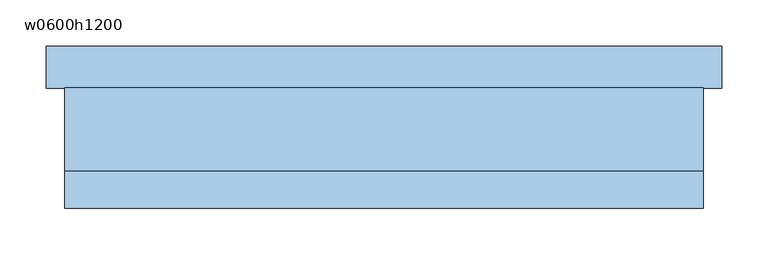
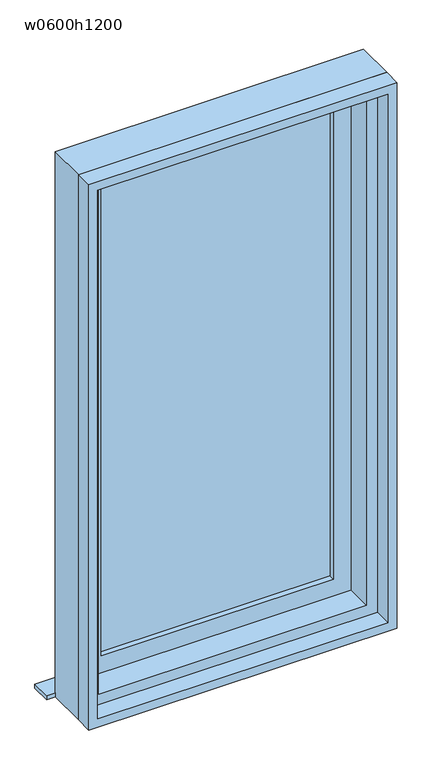
"""IFC4 building model written with IfcOpenShell, lengths in millimetres: window geometry, 縦すべり窓 : w0600h1200."""

from ifc_helpers import new_model, si_unit, frame, origin, place, context, project, spatial, polyline, outline, extrude, source, transform, mapped, element, save


def w0600h1200_ca4a6b53(model_context):
    return source(origin(), model_context, "Body", "SweptSolid", [
        extrude(outline(polyline([(260.0, 27.5), (-260.0, 27.5), (-260.0, 32.5), (260.0, 32.5), (260.0, 27.5)])), frame((0.0, 0.0, 840.0), z_axis=(0.0, 0.0, 1.0), x_axis=(1.0, 0.0, 0.0)), (0.0, 0.0, 1.0), 1120.0),
        extrude(outline(polyline([(2000.0, 300.0), (2000.0, -300.0), (800.0, -300.0), (800.0, 300.0), (2000.0, 300.0)]), holes=[polyline([(1960.0, -260.0), (1960.0, 260.0), (840.0, 260.0), (840.0, -260.0), (1960.0, -260.0)])]), frame((0.0, 15.0, 0.0), z_axis=(0.0, 1.0, 0.0), x_axis=(0.0, 0.0, 1.0)), (0.0, 0.0, 1.0), 30.0),
        extrude(outline(polyline([(365.0, 90.0), (365.0, 45.0), (-365.0, 45.0), (-365.0, 90.0), (365.0, 90.0)])), frame((0.0, 0.0, 755.0), z_axis=(0.0, 0.0, 1.0), x_axis=(1.0, 0.0, 0.0)), (0.0, 0.0, 1.0), 10.0),
        extrude(outline(polyline([(2045.0, 345.0), (2045.0, -345.0), (755.0, -345.0), (755.0, 345.0), (2045.0, 345.0)]), holes=[polyline([(775.0, -325.0), (2025.0, -325.0), (2025.0, 325.0), (775.0, 325.0), (775.0, -325.0)])]), frame((0.0, -85.0, 0.0), z_axis=(0.0, 1.0, 0.0), x_axis=(0.0, 0.0, 1.0)), (0.0, 0.0, 1.0), 40.0),
        extrude(outline(polyline([(2045.0, -345.0), (755.0, -345.0), (755.0, 345.0), (2045.0, 345.0), (2045.0, -345.0)]), holes=[polyline([(2000.0, 300.0), (800.0, 300.0), (800.0, -300.0), (2000.0, -300.0), (2000.0, 300.0)])]), frame((0.0, -45.0, 0.0), z_axis=(0.0, 1.0, 0.0), x_axis=(0.0, 0.0, 1.0)), (0.0, 0.0, 1.0), 90.0),
    ])


if __name__ == "__main__":
    model = new_model("IFC4")
    model_context = context("Model", 3, world=origin())
    ifc_project = project(units=[si_unit("LENGTHUNIT", "METRE", prefix="MILLI")], contexts=[model_context])
    site = spatial("IfcSite", under=ifc_project)
    building = spatial("IfcBuilding", under=site)
    placement = place(None, origin())
    w0600h1200_shape = w0600h1200_ca4a6b53(model_context)
    element("IfcWindow", 1, ObjectType="縦すべり窓 : w0600h1200", at=placement, inside=building, context=model_context, shape_type="MappedRepresentation", body=[
        mapped(w0600h1200_shape, transform((0.0, 0.0, 0.0), x_axis=(1.0, 0.0, 0.0), y_axis=(0.0, 1.0, 0.0), z_axis=(0.0, 0.0, 1.0))),
    ])
    save(model, "model.ifc")

# Revit data of these elements
# Type "縦すべり窓 : w0600h1200"
#   Construction Type Id = "GSP4R"
#   Analytic Construction = "1/8 インチ ピルキントン一重ガラス"
#   Type Mark = "86"
#   Operation = "シングルパネル"
#   Keynote = "08520.S3"
#   Visual Light Transmittance = 0.9
#   Solar Heat Gain Coefficient = 0.86
#   Heat Transfer Coefficient (U) = 6.7069 W/(m²·K)
#   Height = 1200 mm
#   既定の腰高 = 800 mm
#   Width = 600 mm
#   額縁見附 = 20 mm
#   額縁ちり = 10 mm
#   サッシ見附 = 45 mm
#   サッシの幅 = 90 mm
#   サッシ額縁 [instance default] = none
#   サッシ本体 [instance default] = none
#   サッシガラス [instance default] = ガラス - 透明
#   Wall Closure = (empty or 0)
#   Type Comments = ""
#   Assembly Code = ""
# Element 1 (IfcWindow, "縦すべり窓 : w0600h1200")
#   Materials on its faces: "ガラス - 透明"
# Materials
#   "ガラス - 透明": class "ガラス", colour RGB 0 128 192, transparency 0.9, Cost = 0
